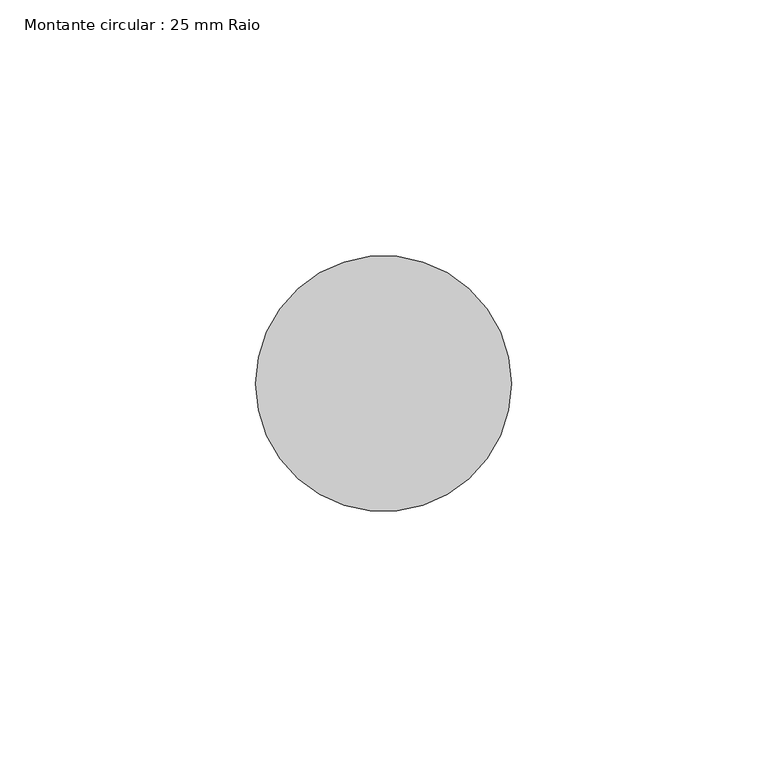
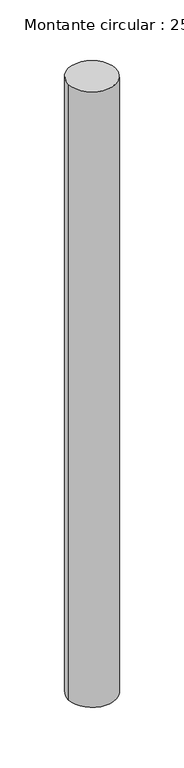
"""IFC4 building model written with IfcOpenShell, lengths in millimetres: member geometry, Montante circular : 25 mm Raio."""

import ifcopenshell
import ifcopenshell.guid

model = None  # the IFC model being written
_history = None  # IfcOwnerHistory: only IFC2X3 demands one
_inside = {}  # id of a spatial element -> (the spatial element, [elements in it])
_under = {}  # id of a project, library or spatial element -> (it, [spatial elements below it])
_declared = {}  # id of a project -> (the project, [libraries it declares])
_typed = {}  # id of a type object -> (the type object, [elements of that type])
_made_of = {}  # id of a material, layer set ... -> (it, [elements and type objects made of it])


def new_model(schema):
    """Start an empty IFC model of exactly this schema.

    Asked for "IFC4X3", IfcOpenShell would pick the latest addendum, in which some entities
    have other attributes; the version numbers below select the first issue.
    IFC2X3 requires an IfcOwnerHistory on every rooted entity: one is made here for all.
    """
    global model, _history
    if schema == "IFC4X3":
        model = ifcopenshell.file(schema_version=(4, 3, 0, 0))
    else:
        model = ifcopenshell.file(schema=schema)
    _inside.clear()
    _under.clear()
    _declared.clear()
    _typed.clear()
    _made_of.clear()
    _history = None
    if model.schema == "IFC2X3":
        org = make("IfcOrganization", Name="unknown")
        user = make(
            "IfcPersonAndOrganization",
            ThePerson=make("IfcPerson", FamilyName="unknown"),
            TheOrganization=org,
        )
        app = make(
            "IfcApplication",
            ApplicationDeveloper=org,
            Version="unknown",
            ApplicationFullName="unknown",
            ApplicationIdentifier="unknown",
        )
        _history = make(
            "IfcOwnerHistory",
            OwningUser=user,
            OwningApplication=app,
            ChangeAction="ADDED",
            CreationDate=0,
        )
    return model


def make(cls, **values):
    """One entity of the class cls with the attributes given. An attribute that is None is left unset."""
    return model.create_entity(
        cls, **{name: value for name, value in values.items() if value is not None}
    )


def rooted(cls, **values):
    """An entity with a GlobalId (a new one), such as an element, a storey or a relation."""
    return make(cls, GlobalId=ifcopenshell.guid.new(), OwnerHistory=_history, **values)


def si_unit(unit_type, name, prefix=None):
    """IfcSIUnit, for example si_unit("LENGTHUNIT", "METRE", prefix="MILLI")."""
    return make("IfcSIUnit", UnitType=unit_type, Prefix=prefix, Name=name)


def assignment(units):
    """IfcUnitAssignment: the units of a project."""
    return None if units is None else make("IfcUnitAssignment", Units=units)


def point(xyz):
    """IfcCartesianPoint."""
    return None if xyz is None else make("IfcCartesianPoint", Coordinates=xyz)


def direction(xyz):
    """IfcDirection."""
    return None if xyz is None else make("IfcDirection", DirectionRatios=xyz)


def frame(location, z_axis=None, x_axis=None):
    """IfcAxis2Placement3D, a coordinate frame: its origin and axes. An axis left out is left unset."""
    return make(
        "IfcAxis2Placement3D",
        Location=point(location),
        Axis=direction(z_axis),
        RefDirection=direction(x_axis),
    )


def frame_2d(location, x_axis=None):
    """IfcAxis2Placement2D, a coordinate frame in the plane: its origin and x axis."""
    return make(
        "IfcAxis2Placement2D", Location=point(location), RefDirection=direction(x_axis)
    )


def origin():
    """The frame at (0, 0, 0) with its axes left unset."""
    return frame((0.0, 0.0, 0.0))


def origin_2d():
    """The frame at (0, 0) in the plane with its x axis left unset."""
    return frame_2d((0.0, 0.0))


def place(relative_to, where):
    """IfcLocalPlacement: puts the frame where relative to a parent placement (None: the world)."""
    return make(
        "IfcLocalPlacement", PlacementRelTo=relative_to, RelativePlacement=where
    )


def context(
    kind, dimensions, precision=None, world=None, true_north=None, identifier=None
):
    """IfcGeometricRepresentationContext, for example the 3D "Model" context."""
    return make(
        "IfcGeometricRepresentationContext",
        ContextIdentifier=identifier,
        ContextType=kind,
        CoordinateSpaceDimension=dimensions,
        Precision=precision,
        WorldCoordinateSystem=world,
        TrueNorth=true_north,
    )


def project(units=None, contexts=None):
    """IfcProject with its units and contexts."""
    return rooted(
        "IfcProject",
        Name="project",
        RepresentationContexts=contexts,
        UnitsInContext=assignment(units),
    )


def spatial(cls, under=None, at=None, **own):
    """A site, building, storey or space (cls), placed at a placement, below another one or the project."""
    s = rooted(cls, ObjectPlacement=at, **own)
    if under is not None:
        _under.setdefault(under.id(), (under, []))[1].append(s)
    return s


def circle_curve(where, radius):
    """IfcCircle in the frame where."""
    return make("IfcCircle", Position=where, Radius=radius)


def trimmed(basis, trim1, trim2, sense, master):
    """IfcTrimmedCurve: the piece of a basis curve between two trims."""
    return make(
        "IfcTrimmedCurve",
        BasisCurve=basis,
        Trim1=trim1,
        Trim2=trim2,
        SenseAgreement=sense,
        MasterRepresentation=master,
    )


def segment(curve, same_sense, transition):
    """IfcCompositeCurveSegment."""
    return make(
        "IfcCompositeCurveSegment",
        Transition=transition,
        SameSense=same_sense,
        ParentCurve=curve,
    )


def composite_curve(segments, self_intersect=None):
    """IfcCompositeCurve: segments joined end to end."""
    return make("IfcCompositeCurve", Segments=segments, SelfIntersect=self_intersect)


def outline(outer, holes=None, kind="AREA"):
    """IfcArbitraryClosedProfileDef: a profile drawn as a closed curve; with holes, ...WithVoids."""
    if holes is None:
        return make("IfcArbitraryClosedProfileDef", ProfileType=kind, OuterCurve=outer)
    return make(
        "IfcArbitraryProfileDefWithVoids",
        ProfileType=kind,
        OuterCurve=outer,
        InnerCurves=holes,
    )


def extrude(swept, where, along, depth):
    """IfcExtrudedAreaSolid: the profile swept, set in the frame where, extruded along a direction by depth."""
    return make(
        "IfcExtrudedAreaSolid",
        SweptArea=swept,
        Position=where,
        ExtrudedDirection=direction(along),
        Depth=depth,
    )


def shape(context_of_items, identifier, shape_type, items):
    """IfcShapeRepresentation: the items that make up one representation, for example the "Body"."""
    return make(
        "IfcShapeRepresentation",
        ContextOfItems=context_of_items,
        RepresentationIdentifier=identifier,
        RepresentationType=shape_type,
        Items=items,
    )


def source(mapping_origin, context_of_items, identifier, shape_type, items):
    """IfcRepresentationMap: a shape defined once, which mapped items show again and again."""
    return make(
        "IfcRepresentationMap",
        MappingOrigin=mapping_origin,
        MappedRepresentation=shape(context_of_items, identifier, shape_type, items),
    )


def transform(
    local_origin,
    x_axis=None,
    y_axis=None,
    z_axis=None,
    scale=None,
    scale2=None,
    scale3=None,
    uniform=True,
):
    """IfcCartesianTransformationOperator3D, or its non-uniform kind. x_axis, y_axis, z_axis: its Axis1, 2, 3."""
    if uniform:
        return make(
            "IfcCartesianTransformationOperator3D",
            Axis1=direction(x_axis),
            Axis2=direction(y_axis),
            LocalOrigin=point(local_origin),
            Scale=scale,
            Axis3=direction(z_axis),
        )
    return make(
        "IfcCartesianTransformationOperator3DnonUniform",
        Axis1=direction(x_axis),
        Axis2=direction(y_axis),
        LocalOrigin=point(local_origin),
        Scale=scale,
        Axis3=direction(z_axis),
        Scale2=scale2,
        Scale3=scale3,
    )


def mapped(mapping_source, mapping_target):
    """IfcMappedItem: shows the shape of a source again, moved by a transform."""
    return make(
        "IfcMappedItem", MappingSource=mapping_source, MappingTarget=mapping_target
    )


def made_of(thing, what):
    """Note that an element or type object is made of a material, layer set ...; save() writes the relation."""
    if what is not None:
        _made_of.setdefault(what.id(), (what, []))[1].append(thing)
    return thing


def element(
    cls,
    number,
    at=None,
    inside=None,
    cuts=None,
    type_object=None,
    material=None,
    context=None,
    identifier="Body",
    shape_type=None,
    held_by="IfcProductDefinitionShape",
    body=None,
    shapes=None,
    **own,
):
    """One element of the class cls, such as IfcWall. Its Tag is "e" and its number.

    at: its placement. inside: the storey or other place that contains it. cuts: it is an
    opening in that element (IfcRelVoidsElement). A single representation is given by context,
    identifier, shape_type and body (its items); several are given by shapes. held_by: the class
    of the entity that holds the representations. save() writes the other relations.
    """
    e = rooted(cls, Tag="e%d" % number, ObjectPlacement=at, **own)
    if body is not None:
        shapes = [shape(context, identifier, shape_type, body)]
    if shapes is not None:
        e.Representation = make(held_by, Representations=shapes)
    if inside is not None:
        _inside.setdefault(inside.id(), (inside, []))[1].append(e)
    if cuts is not None:
        rooted(
            "IfcRelVoidsElement", RelatingBuildingElement=cuts, RelatedOpeningElement=e
        )
    if type_object is not None:
        _typed.setdefault(type_object.id(), (type_object, []))[1].append(e)
    return made_of(e, material)


def aggregate(whole, parts):
    """IfcRelAggregates: a whole, such as a stair, and the parts it consists of."""
    return rooted("IfcRelAggregates", RelatingObject=whole, RelatedObjects=parts)


def save(model, path):
    """Write the relations noted so far, then the file.

    IfcRelAggregates (storeys below a building ...), IfcRelContainedInSpatialStructure (elements
    in a storey), IfcRelDefinesByType, IfcRelAssociatesMaterial and IfcRelDeclares: one each for
    every whole, place, type object, material and project.
    """
    for whole, parts in _under.values():
        aggregate(whole, parts)
    for where, things in _inside.values():
        rooted(
            "IfcRelContainedInSpatialStructure",
            RelatedElements=things,
            RelatingStructure=where,
        )
    for kind, things in _typed.values():
        rooted("IfcRelDefinesByType", RelatedObjects=things, RelatingType=kind)
    for what, things in _made_of.values():
        rooted("IfcRelAssociatesMaterial", RelatedObjects=things, RelatingMaterial=what)
    for by, libraries in _declared.values():
        rooted("IfcRelDeclares", RelatingContext=by, RelatedDefinitions=libraries)
    model.write(path)


def montante_circular_25_mm_raio_b6a72e74(model_context):
    return source(origin(), model_context, "Body", "SweptSolid", [
        extrude(outline(composite_curve([segment(trimmed(circle_curve(origin_2d(), 25.0), [point((25.0, 0.0))], [point((-25.0, 0.0))], False, "CARTESIAN"), True, "CONTINUOUS"), segment(trimmed(circle_curve(origin_2d(), 25.0), [point((-25.0, 0.0))], [point((25.0, 0.0))], False, "CARTESIAN"), True, "CONTINUOUS")], self_intersect=False)), frame((0.0, 0.0, -685.7133319), z_axis=(0.0, 0.0, 1.0), x_axis=(1.0, 0.0, 0.0)), (0.0, 0.0, 1.0), 685.7133319),
    ])


if __name__ == "__main__":
    model = new_model("IFC4")
    model_context = context("Model", 3, world=origin())
    ifc_project = project(units=[si_unit("LENGTHUNIT", "METRE", prefix="MILLI")], contexts=[model_context])
    site = spatial("IfcSite", under=ifc_project)
    building = spatial("IfcBuilding", under=site)
    placement = place(None, origin())
    montante_circular_25_mm_raio_shape = montante_circular_25_mm_raio_b6a72e74(model_context)
    element("IfcMember", 1, ObjectType="Montante circular : 25 mm Raio", at=placement, inside=building, context=model_context, shape_type="MappedRepresentation", body=[
        mapped(montante_circular_25_mm_raio_shape, transform((0.0, 0.0, 0.0), x_axis=(1.0, 0.0, 0.0), y_axis=(0.0, 1.0, 0.0), z_axis=(0.0, 0.0, 1.0))),
    ])
    save(model, "model.ifc")

# Revit data of these elements
# Type "Montante circular : 25 mm Raio"
#   built-in parameter 1007350 = 0.082021 (stored number, unit not read)
# Element 1 (IfcMember, "Montante circular : 25 mm Raio")
#   Materials on its faces: "Alumín."
# Materials
#   "Alumín.": class "Metal", colour RGB 247 247 247, transparency 0, Description = "Alumín. 6061", Cost = 0
